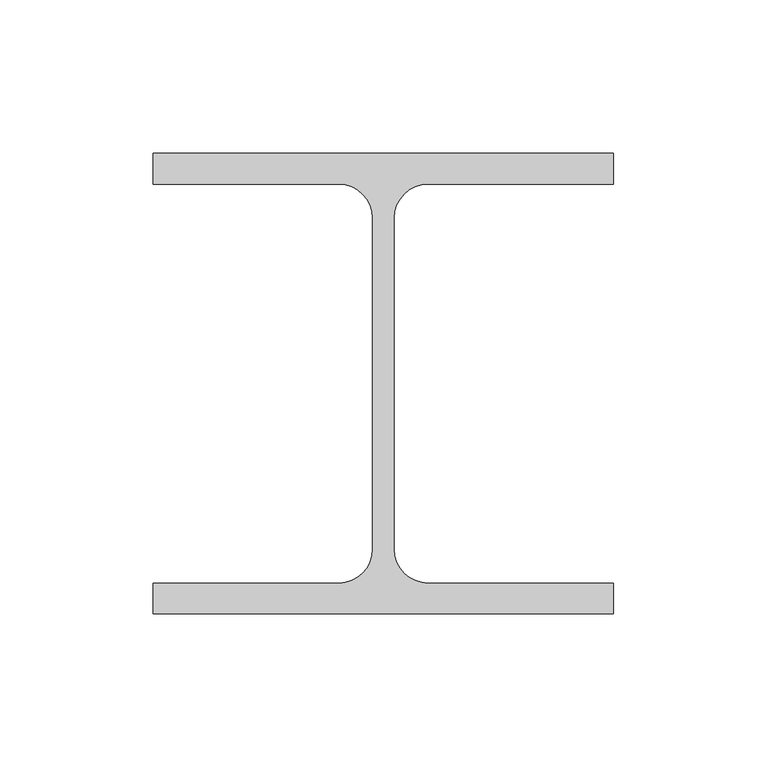
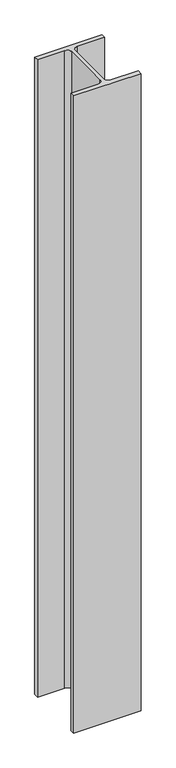
"""IFC4 building model written with IfcOpenShell, lengths in millimetres: column geometry, 0912_Steel Column_H_KSD3502 : H_SC_ASC_H-150x150x7x10."""

from ifc_helpers import new_model, si_unit, point, frame, frame_2d, origin, place, context, project, spatial, polyline, circle_curve, trimmed, segment, composite_curve, outline, extrude, source, transform, mapped, element, save


def column_0d301b3b(model_context):
    return source(origin(), model_context, "Body", "SweptSolid", [
        extrude(outline(composite_curve([segment(polyline([(75.0, 75.0), (75.0, 65.0), (14.5, 65.0)]), True, "CONTINUOUS"), segment(trimmed(circle_curve(frame_2d((14.5, 54.0)), 11.0), [point((14.5, 65.0))], [point((3.5, 54.0))], True, "CARTESIAN"), True, "CONTINUOUS"), segment(polyline([(3.5, 54.0), (3.5, -54.0)]), True, "CONTINUOUS"), segment(trimmed(circle_curve(frame_2d((14.5, -54.0)), 11.0), [point((3.5, -54.0))], [point((14.5, -65.0))], True, "CARTESIAN"), True, "CONTINUOUS"), segment(polyline([(14.5, -65.0), (75.0, -65.0), (75.0, -75.0), (-75.0, -75.0), (-75.0, -65.0), (-14.5, -65.0)]), True, "CONTINUOUS"), segment(trimmed(circle_curve(frame_2d((-14.5, -54.0)), 11.0), [point((-14.5, -65.0))], [point((-3.5, -54.0))], True, "CARTESIAN"), True, "CONTINUOUS"), segment(polyline([(-3.5, -54.0), (-3.5, 54.0)]), True, "CONTINUOUS"), segment(trimmed(circle_curve(frame_2d((-14.5, 54.0)), 11.0), [point((-3.5, 54.0))], [point((-14.5, 65.0))], True, "CARTESIAN"), True, "CONTINUOUS"), segment(polyline([(-14.5, 65.0), (-75.0, 65.0), (-75.0, 75.0), (75.0, 75.0)]), True, "CONTINUOUS")], self_intersect=False)), frame((0.0, 0.0, 6299.9720055), z_axis=(0.0, 0.0, 1.0), x_axis=(1.0, 0.0, 0.0)), (0.0, 0.0, 1.0), 1500.0),
    ])


if __name__ == "__main__":
    model = new_model("IFC4")
    model_context = context("Model", 3, world=origin())
    ifc_project = project(units=[si_unit("LENGTHUNIT", "METRE", prefix="MILLI")], contexts=[model_context])
    site = spatial("IfcSite", under=ifc_project)
    building = spatial("IfcBuilding", under=site)
    placement = place(None, origin())
    column_shape = column_0d301b3b(model_context)
    element("IfcColumn", 1, ObjectType="0912_Steel Column_H_KSD3502 : H_SC_ASC_H-150x150x7x10", at=placement, inside=building, context=model_context, shape_type="MappedRepresentation", body=[
        mapped(column_shape, transform((0.0, 0.0, 0.0), x_axis=(1.0, 0.0, 0.0), y_axis=(0.0, 1.0, 0.0), z_axis=(0.0, 0.0, 1.0))),
    ])
    save(model, "model.ifc")

# Revit data of these elements
# Type "0912_Steel Column_H_KSD3502 : H_SC_ASC_H-150x150x7x10"
#   H_WM Code_1 = "S01AA002-00001 | Main Steel Structure Fabrication Work | Shelter/Building | Medium Steel - Standard (90KG/M>Weight≥30KG/M) | Material: (   )"
#   H_WM Code_2 = "S03AA028-00001 | Main Steel Structure Erection Work | Shelter/Building | Medium Steel (90KG/M>Weight≥30KG/M) | Material: (   )"
#   H_WM Code_3 = "S01AA010-00001 | Main Steel Structure Fabrication Work | Shelter/Building | Steel Painting/Coating | for Non-Fireproofed Steel Surface, Surface Preparation, Primer, Second & Final Coat | Material: (   )"
#   H_Q'ty Cal Type Tag = "SC-Q2"
#   Width = 15.0 cm
#   Web Thickness = 0.7 cm
#   Web Fillet = 1.1 cm
#   Warping Constant = 27562.5 cm⁶
#   Torsional Moment of Inertia = 11.6007 cm⁴
#   Section Area = 40.14 cm²
#   Plastic Modulus weak axis = 115.0 cm³
#   Plastic Modulus strong axis = 246.0 cm³
#   Perimeter = 0.87 m²/m
#   Nominal Weight = 31.50 kgf/m
#   Moment of Inertia weak axis = 563.00 cm⁴
#   Moment of Inertia strong axis = 1640.00 cm⁴
#   Height = 15.0 cm
#   Flange Thickness = 1.0 cm
#   Elastic Modulus weak axis = 75.1 cm³
#   Elastic Modulus strong axis = 219.0 cm³
#   Centroid Vertical = 7.5 cm
#   Centroid Horizontal = 7.5 cm
#   Structural Material [instance default] = Steel, 45-345
#   Section Name Key = ""
#   Bolt Spacing = 0
#   Assembly Code = ""
# Element 1 (IfcColumn, "0912_Steel Column_H_KSD3502 : H_SC_ASC_H-150x150x7x10")
#   Structural Material = none
# Materials
#   "Steel, 45-345": class "Metal", colour RGB 189 187 185, transparency 0, Description = "Steel 345 MPa", Cost = 0
